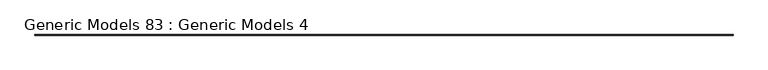
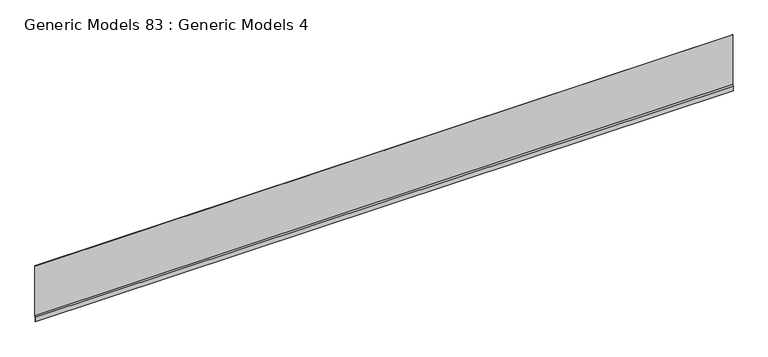
"""IFC4 building model written with IfcOpenShell, lengths in millimetres: proxy geometry, Generic Models 83 : Generic Models 4."""

from ifc_helpers import new_model, si_unit, frame, origin, place, context, project, spatial, polyline, outline, extrude, source, transform, mapped, element, save


def generic_models_83_generic_models_4_ecc62c31(model_context):
    return source(origin(), model_context, "Body", "SweptSolid", [
        extrude(outline(polyline([(-7075.2700728, 123464.3768419), (-7079.9031787, 123451.647488), (-7079.9031787, 123410.1798411), (-7080.6969287, 123410.1798411), (-7080.6969287, 123451.7874476), (-7076.0638228, 123464.5168015), (-7076.0638228, 123930.164006), (-7075.2700728, 123930.164006), (-7075.2700728, 123464.3768419)])), frame((2196.9263704, 0.0, 0.0), z_axis=(1.0, 0.0, 0.0), x_axis=(0.0, 1.0, 0.0)), (0.0, 0.0, 1.0), 6212.156498),
    ])


if __name__ == "__main__":
    model = new_model("IFC4")
    model_context = context("Model", 3, world=origin())
    ifc_project = project(units=[si_unit("LENGTHUNIT", "METRE", prefix="MILLI")], contexts=[model_context])
    site = spatial("IfcSite", under=ifc_project)
    building = spatial("IfcBuilding", under=site)
    placement = place(None, origin())
    generic_models_83_generic_models_4_shape = generic_models_83_generic_models_4_ecc62c31(model_context)
    element("IfcBuildingElementProxy", 1, Name="Generic Models 83 : Generic Models 4", ObjectType="Generic Models 83 : Generic Models 4", at=placement, inside=building, context=model_context, shape_type="MappedRepresentation", body=[
        mapped(generic_models_83_generic_models_4_shape, transform((0.0, 0.0, 0.0), x_axis=(1.0, 0.0, 0.0), y_axis=(0.0, 1.0, 0.0), z_axis=(0.0, 0.0, 1.0))),
    ])
    save(model, "model.ifc")

# Revit data of these elements
# Element 1 (IfcBuildingElementProxy, "Generic Models 83 : Generic Models 4")
#   Materials on its faces: "_(2) LAYERS NO. 30 ASTM D226 ASPHALT SATURATED ORGANIC FELT"
# Materials
#   "_(2) LAYERS NO. 30 ASTM D226 ASPHALT SATURATED ORGANIC FELT": class "Generic", colour RGB 67 154 161, transparency 0, Cost = 0
